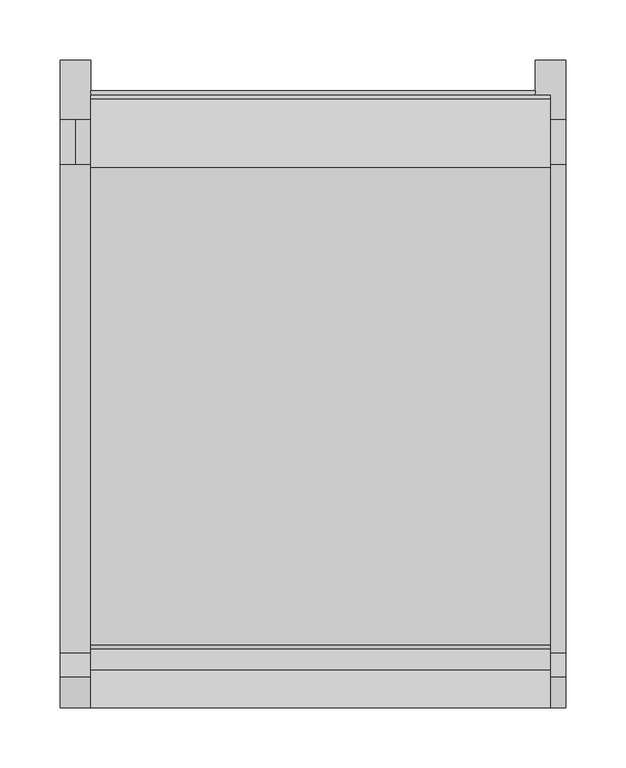
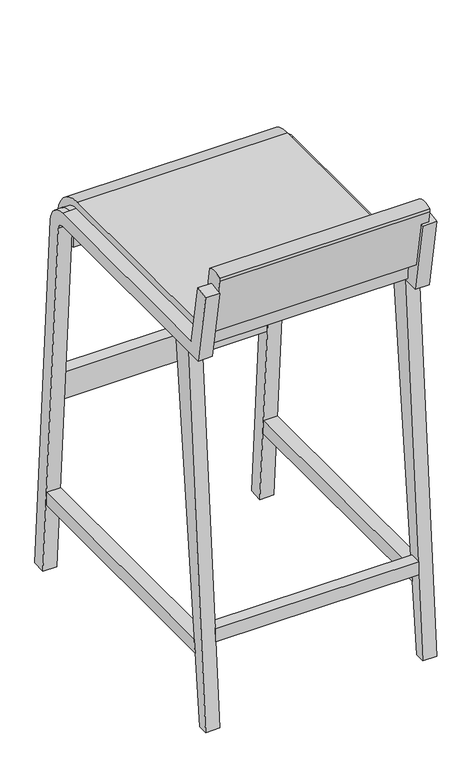
"""IFC4 building model written with IfcOpenShell, lengths in millimetres: furniture geometry, Bar_Stool_6722[1] : Bar_Stool_6722[1]."""

from ifc_helpers import new_model, si_unit, point, frame, frame_2d, origin, place, context, project, spatial, polyline, circle_curve, trimmed, segment, composite_curve, outline, extrude, source, transform, mapped, element, save
from ifc_brep_helpers import plane_surface, cylinder_surface, revolved_surface, advanced_brep


def furniture_48a66dd3(model_context):
    return source(origin(), model_context, "Body", "SolidModel", [
        advanced_brep(
        [(419.1, 25.0141169, 838.4759165), (393.7, 25.0141169, 838.4759165), (393.7, 0.0, 834.0652528), (419.1, 0.0, 834.0652528), (419.1, 45.2169423, 723.9), (393.7, 45.2169423, 723.9), (393.7, 450.0350637, 723.9), (393.7, 488.0397183, 688.4937383), (393.7, 536.7759384, 0.8979128), (393.7, 511.439502, -0.8979128), (393.7, 462.7032819, 686.6979128), (393.7, 450.0350637, 698.5), (393.7, 23.9038117, 698.5), (419.1, 23.9038117, 698.5), (419.1, 450.0350637, 698.5), (419.1, 462.7032819, 686.6979128), (419.1, 511.439502, -0.8979128), (419.1, 536.7759384, 0.8979128), (419.1, 488.0397183, 688.4937383), (419.1, 450.0350637, 723.9), (406.4, 450.0350637, 723.9), (406.4, 488.0397183, 688.4937383)],
        [
            (0, 1),
            (1, 2),
            (2, 3),
            (3, 0),
            (0, 4),
            (4, 5),
            (5, 1),
            (5, 6),
            (6, 7, circle_curve(frame((393.7, 450.0350637, 685.8), z_axis=(-1.0, 0.0, 0.0), x_axis=(0.0, 0.0, 1.0)), 38.1)),
            (7, 8),
            (8, 9),
            (9, 10),
            (10, 11, circle_curve(frame((393.7, 450.0350637, 685.8), z_axis=(1.0, 0.0, 0.0), x_axis=(0.0, 0.0, 1.0)), 12.7)),
            (11, 12),
            (12, 2),
            (12, 13),
            (13, 3),
            (13, 14),
            (14, 15, circle_curve(frame((419.1, 450.0350637, 685.8), z_axis=(-1.0, 0.0, 0.0), x_axis=(0.0, 0.0, 1.0)), 12.7)),
            (15, 16),
            (16, 17),
            (17, 18),
            (18, 19, circle_curve(frame((419.1, 450.0350637, 685.8), z_axis=(1.0, 0.0, 0.0), x_axis=(0.0, 0.0, 1.0)), 38.1)),
            (19, 4),
            (19, 20),
            (20, 6),
            (11, 14),
            (21, 20, circle_curve(frame((406.4, 450.0350637, 685.8), z_axis=(1.0, 0.0, 0.0), x_axis=(0.0, 0.0, 1.0)), 38.1)),
            (18, 21),
            (21, 7),
            (10, 15),
            (17, 8),
            (9, 16),
        ],
        [
            plane_surface(frame((406.4, 12.5070585, 836.2705846), z_axis=(0.0, -0.17364817766692853, 0.9848077530122085), x_axis=(1.0, 0.0, 0.0))),
            plane_surface(frame((406.4, 25.0141169, 838.4759165), z_axis=(0.0, 0.9848077530122085, 0.17364817766692814), x_axis=(0.0, 0.17364817766692814, -0.9848077530122085))),
            plane_surface(frame((393.7, 25.0141169, 838.4759165), z_axis=(-1.0, 0.0, 0.0), x_axis=(0.0, 0.17364817766692808, -0.9848077530122085))),
            plane_surface(frame((393.7, 0.0, 834.0652528), z_axis=(0.0, -0.9848077530122085, -0.17364817766692817), x_axis=(0.0, 0.17364817766692817, -0.9848077530122085))),
            plane_surface(frame((419.1, 0.0, 834.0652528), z_axis=(1.0000000000000002, 0.0, 0.0), x_axis=(0.0, 0.1736481776669284, -0.9848077530122085))),
            plane_surface(frame((406.4, 45.2169423, 723.9), z_axis=(0.0, 0.0, 1.0), x_axis=(0.0, 1.0, 0.0))),
            plane_surface(frame((393.7, 23.9038117, 698.5), z_axis=(0.0, 0.0, -1.0), x_axis=(0.0, 1.0, 0.0))),
            cylinder_surface(frame((406.4, 450.0350637, 685.8), z_axis=(-1.0, 0.0, 0.0), x_axis=(0.0, 0.0, 1.0)), 38.1),
            revolved_surface(polyline([(393.7, 450.0350637, 698.5), (419.1, 450.0350637, 698.5)]), (406.4, 450.0350637, 685.8), (-1.0, 0.0, 0.0)),
            plane_surface(frame((406.4, 488.0397183, 688.4937383), z_axis=(0.0, 0.9974974969901172, 0.07070179275273744), x_axis=(0.0, 0.07070179275273744, -0.9974974969901172))),
            plane_surface(frame((393.7, 462.7032819, 686.6979128), z_axis=(0.0, -0.9974974969901172, -0.07070179275273743), x_axis=(0.0, 0.07070179275273743, -0.9974974969901172))),
            plane_surface(frame((406.4, 524.1077202, 0.0), z_axis=(0.0, 0.07070179275273399, -0.9974974969901175), x_axis=(1.0, 0.0, 0.0))),
        ],
        [
            (0, [[1, 2, 3, 4]]),
            (1, [[5, 6, 7, -1]]),
            (2, [[-2, -7, 8, 9, 10, 11, 12, 13, 14, 15]]),
            (3, [[-3, -15, 16, 17]]),
            (4, [[-4, -17, 18, 19, 20, 21, 22, 23, 24, -5]]),
            (5, [[-6, -24, 25, 26, -8]]),
            (6, [[-16, -14, 27, -18]]),
            (7, [[28, -25, -23, 29]]),
            (7, [[-9, -26, -28, 30]]),
            (8, [[-19, -27, -13, 31]]),
            (9, [[-10, -30, -29, -22, 32]]),
            (10, [[-20, -31, -12, 33]]),
            (11, [[-32, -21, -33, -11]]),
        ],
    ),
        extrude(outline(composite_curve([segment(polyline([(48.4096386, 756.5644068), (44.0710693, 752.2258375), (19.1416957, 748.2774126), (0.0, 856.8353632), (0.0, 863.1853632)]), True, "CONTINUOUS"), segment(trimmed(circle_curve(frame_2d((15.7612691, 828.3540875)), 38.2313401), [point((0.0, 863.1853632))], [point((31.5225381, 863.1853632))], False, "CARTESIAN"), True, "CONTINUOUS"), segment(polyline([(31.5225381, 863.1853632), (48.4096386, 756.5644068)]), True, "CONTINUOUS")], self_intersect=False)), frame((25.4, 0.0, 0.0), z_axis=(1.0, 0.0, 0.0), x_axis=(0.0, 1.0, 0.0)), (0.0, 0.0, 1.0), 381.0),
        extrude(outline(composite_curve([segment(polyline([(51.6744261, 737.5144068), (447.8968201, 737.5144068)]), True, "CONTINUOUS"), segment(trimmed(circle_curve(frame_2d((447.8968201, 676.6245275)), 60.8898793), [point((447.8968201, 737.5144068))], [point((505.1145904, 697.4500928))], False, "CARTESIAN"), True, "CONTINUOUS"), segment(trimmed(circle_curve(frame_2d((460.5585493, 681.23302)), 47.4155486), [point((505.1145904, 697.4500928))], [point((484.2663236, 640.1699505))], False, "CARTESIAN"), True, "CONTINUOUS"), segment(polyline([(484.2663236, 640.1699505), (460.5585493, 643.13302), (460.5585493, 681.23302), (452.817441, 704.85), (46.417441, 704.85), (43.9498561, 733.0546243), (51.6744261, 737.5144068)]), True, "CONTINUOUS")], self_intersect=False)), frame((25.4, 0.0, 0.0), z_axis=(1.0, 0.0, 0.0), x_axis=(0.0, 1.0, 0.0)), (0.0, 0.0, 1.0), 381.0),
        extrude(outline(polyline([(393.7, 11.6871233), (25.4, 11.6871233), (25.4, 33.1441574), (393.7, 33.1441574), (393.7, 11.6871233)])), frame((0.0, 0.0, 157.9619127), z_axis=(0.0, 0.0, 1.0), x_axis=(1.0, 0.0, 0.0)), (0.0, 0.0, 1.0), 25.4),
        extrude(outline(polyline([(393.7, 488.2695397), (25.4, 488.2695397), (25.4, 511.439502), (393.7, 511.439502), (393.7, 488.2695397)])), frame((0.0, 0.0, 335.7619127), z_axis=(0.0, 0.0, 1.0), x_axis=(1.0, 0.0, 0.0)), (0.0, 0.0, 1.0), 50.8),
        extrude(outline(polyline([(500.1796497, 157.9619127), (500.1796497, 132.5619127), (32.9828185, 132.5619127), (35.652466, 157.9619127), (500.1796497, 157.9619127)])), frame((393.7, 0.0, 0.0), z_axis=(1.0, 0.0, 0.0), x_axis=(0.0, 1.0, 0.0)), (0.0, 0.0, 1.0), 25.4),
        extrude(outline(polyline([(500.1796497, 157.9619127), (500.1796497, 132.5619127), (32.9828185, 132.5619127), (35.652466, 157.9619127), (500.1796497, 157.9619127)])), frame((0.0, 0.0, 0.0), z_axis=(1.0, 0.0, 0.0), x_axis=(0.0, 1.0, 0.0)), (0.0, 0.0, 1.0), 25.4),
        extrude(outline(polyline([(0.0, 0.0), (55.3031462, 698.5), (92.4653083, 698.5), (19.05, 0.0), (0.0, 0.0)])), frame((393.7, 0.0, 0.0), z_axis=(1.0, 0.0, 0.0), x_axis=(0.0, 1.0, 0.0)), (0.0, 0.0, 1.0), 25.4),
        advanced_brep(
        [(25.4, 25.0141169, 838.4759165), (0.0, 25.0141169, 838.4759165), (0.0, 0.0, 834.0652528), (25.4, 0.0, 834.0652528), (25.4, 45.2169423, 723.9), (0.0, 45.2169423, 723.9), (0.0, 450.0350637, 723.9), (0.0, 488.0397183, 688.4937383), (0.0, 536.7759384, 0.8979128), (0.0, 511.439502, -0.8979128), (0.0, 462.7032819, 686.6979128), (0.0, 450.0350637, 698.5), (0.0, 23.9038117, 698.5), (25.4, 23.9038117, 698.5), (25.4, 450.0350637, 698.5), (25.4, 462.7032819, 686.6979128), (25.4, 511.439502, -0.8979128), (25.4, 536.7759384, 0.8979128), (25.4, 488.0397183, 688.4937383), (25.4, 450.0350637, 723.9), (12.7, 450.0350637, 723.9), (12.7, 488.0397183, 688.4937383)],
        [
            (0, 1),
            (1, 2),
            (2, 3),
            (3, 0),
            (0, 4),
            (4, 5),
            (5, 1),
            (5, 6),
            (6, 7, circle_curve(frame((0.0, 450.0350637, 685.8), z_axis=(-1.0, 0.0, 0.0), x_axis=(0.0, 0.0, 1.0)), 38.1)),
            (7, 8),
            (8, 9),
            (9, 10),
            (10, 11, circle_curve(frame((0.0, 450.0350637, 685.8), z_axis=(1.0, 0.0, 0.0), x_axis=(0.0, 0.0, 1.0)), 12.7)),
            (11, 12),
            (12, 2),
            (12, 13),
            (13, 3),
            (13, 14),
            (14, 15, circle_curve(frame((25.4, 450.0350637, 685.8), z_axis=(-1.0, 0.0, 0.0), x_axis=(0.0, 0.0, 1.0)), 12.7)),
            (15, 16),
            (16, 17),
            (17, 18),
            (18, 19, circle_curve(frame((25.4, 450.0350637, 685.8), z_axis=(1.0, 0.0, 0.0), x_axis=(0.0, 0.0, 1.0)), 38.1)),
            (19, 4),
            (19, 20),
            (20, 6),
            (11, 14),
            (21, 20, circle_curve(frame((12.7, 450.0350637, 685.8), z_axis=(1.0, 0.0, 0.0), x_axis=(0.0, 0.0, 1.0)), 38.1)),
            (18, 21),
            (21, 7),
            (10, 15),
            (17, 8),
            (9, 16),
        ],
        [
            plane_surface(frame((12.7, 12.5070585, 836.2705846), z_axis=(0.0, -0.17364817766692853, 0.9848077530122085), x_axis=(1.0, 0.0, 0.0))),
            plane_surface(frame((12.7, 25.0141169, 838.4759165), z_axis=(0.0, 0.9848077530122085, 0.173648177666928), x_axis=(0.0, 0.173648177666928, -0.9848077530122085))),
            plane_surface(frame((0.0, 25.0141169, 838.4759165), z_axis=(-1.0, 0.0, 0.0), x_axis=(0.0, 0.17364817766692875, -0.9848077530122084))),
            plane_surface(frame((0.0, 0.0, 834.0652528), z_axis=(0.0, -0.9848077530122084, -0.17364817766692883), x_axis=(0.0, 0.17364817766692883, -0.9848077530122084))),
            plane_surface(frame((25.4, 0.0, 834.0652528), z_axis=(1.0000000000000002, 0.0, 0.0), x_axis=(0.0, 0.1736481776669284, -0.9848077530122085))),
            plane_surface(frame((12.7, 45.2169423, 723.9), z_axis=(0.0, 0.0, 1.0), x_axis=(0.0, 1.0, 0.0))),
            plane_surface(frame((0.0, 23.9038117, 698.5), z_axis=(0.0, 0.0, -1.0), x_axis=(0.0, 1.0, 0.0))),
            cylinder_surface(frame((12.7, 450.0350637, 685.8), z_axis=(-1.0, 0.0, 0.0), x_axis=(0.0, 0.0, 1.0)), 38.1),
            revolved_surface(polyline([(0.0, 450.0350637, 698.5), (25.4, 450.0350637, 698.5)]), (12.7, 450.0350637, 685.8), (-1.0, 0.0, 0.0)),
            plane_surface(frame((12.7, 488.0397183, 688.4937383), z_axis=(0.0, 0.9974974969901172, 0.07070179275273744), x_axis=(0.0, 0.07070179275273744, -0.9974974969901172))),
            plane_surface(frame((0.0, 462.7032819, 686.6979128), z_axis=(0.0, -0.9974974969901172, -0.07070179275273743), x_axis=(0.0, 0.07070179275273743, -0.9974974969901172))),
            plane_surface(frame((12.7, 524.1077202, 0.0), z_axis=(0.0, 0.07070179275273399, -0.9974974969901175), x_axis=(1.0, 0.0, 0.0))),
        ],
        [
            (0, [[1, 2, 3, 4]]),
            (1, [[5, 6, 7, -1]]),
            (2, [[-2, -7, 8, 9, 10, 11, 12, 13, 14, 15]]),
            (3, [[-3, -15, 16, 17]]),
            (4, [[-4, -17, 18, 19, 20, 21, 22, 23, 24, -5]]),
            (5, [[-6, -24, 25, 26, -8]]),
            (6, [[-16, -14, 27, -18]]),
            (7, [[28, -25, -23, 29]]),
            (7, [[-9, -26, -28, 30]]),
            (8, [[-19, -27, -13, 31]]),
            (9, [[-10, -30, -29, -22, 32]]),
            (10, [[-20, -31, -12, 33]]),
            (11, [[-32, -21, -33, -11]]),
        ],
    ),
        extrude(outline(polyline([(0.0, 0.0), (55.3031462, 698.5), (92.4653083, 698.5), (19.05, 0.0), (0.0, 0.0)])), frame((0.0, 0.0, 0.0), z_axis=(1.0, 0.0, 0.0), x_axis=(0.0, 1.0, 0.0)), (0.0, 0.0, 1.0), 25.4),
    ])


if __name__ == "__main__":
    model = new_model("IFC4")
    model_context = context("Model", 3, world=origin())
    ifc_project = project(units=[si_unit("LENGTHUNIT", "METRE", prefix="MILLI")], contexts=[model_context])
    site = spatial("IfcSite", under=ifc_project)
    building = spatial("IfcBuilding", under=site)
    placement = place(None, origin())
    furniture_shape = furniture_48a66dd3(model_context)
    element("IfcFurniture", 1, ObjectType="Bar_Stool_6722[1] : Bar_Stool_6722[1]", at=placement, inside=building, context=model_context, shape_type="MappedRepresentation", body=[
        mapped(furniture_shape, transform((0.0, 0.0, 0.0), x_axis=(1.0, 0.0, 0.0), y_axis=(0.0, 1.0, 0.0), z_axis=(0.0, 0.0, 1.0))),
    ])
    save(model, "model.ifc")

# Revit data of these elements
# Type "Bar_Stool_6722[1] : Bar_Stool_6722[1]"
#   Seat = fab
#   Chair Legs = MET
# Element 1 (IfcFurniture, "Bar_Stool_6722[1] : Bar_Stool_6722[1]")
#   Materials on its faces: "MET", "fab"
# Materials
#   "fab": class "Leather", colour RGB 255 255 255, transparency 0, Cost = 0
#   "MET": class "Metal", colour RGB 189 187 185, transparency 0
